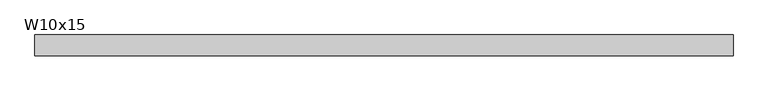
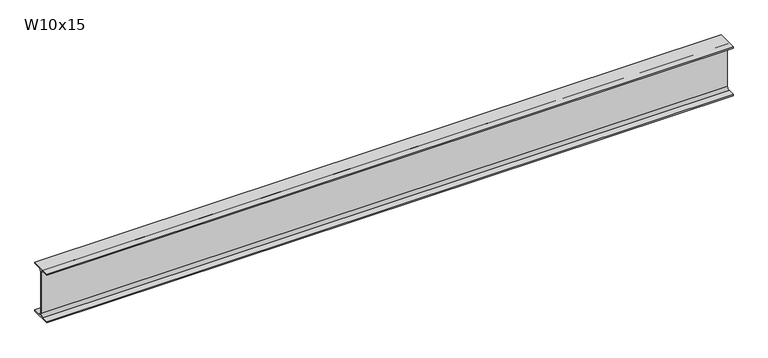
"""IFC4 building model written with IfcOpenShell, lengths in millimetres: beam geometry, RME W-Wide Flange : W10x15."""

from ifc_helpers import new_model, si_unit, point, frame, frame_2d, origin, place, context, project, spatial, polyline, circle_curve, trimmed, segment, composite_curve, outline, extrude, source, transform, mapped, element, save


def w10x15_0be6c648(model_context):
    return source(origin(), model_context, "Body", "SweptSolid", [
        extrude(outline(composite_curve([segment(polyline([(50.8, -120.142), (50.8, -127.0), (-50.8, -127.0), (-50.8, -120.142), (-16.7005, -120.142)]), True, "CONTINUOUS"), segment(trimmed(circle_curve(frame_2d((-16.7005, -106.3625)), 13.7795), [point((-16.7005, -120.142))], [point((-2.921, -106.3625))], True, "CARTESIAN"), True, "CONTINUOUS"), segment(polyline([(-2.921, -106.3625), (-2.921, 106.3625)]), True, "CONTINUOUS"), segment(trimmed(circle_curve(frame_2d((-16.7005, 106.3625)), 13.7795), [point((-2.921, 106.3625))], [point((-16.7005, 120.142))], True, "CARTESIAN"), True, "CONTINUOUS"), segment(polyline([(-16.7005, 120.142), (-50.8, 120.142), (-50.8, 127.0), (50.8, 127.0), (50.8, 120.142), (16.7005, 120.142)]), True, "CONTINUOUS"), segment(trimmed(circle_curve(frame_2d((16.7005, 106.3625)), 13.7795), [point((16.7005, 120.142))], [point((2.921, 106.3625))], True, "CARTESIAN"), True, "CONTINUOUS"), segment(polyline([(2.921, 106.3625), (2.921, -106.3625)]), True, "CONTINUOUS"), segment(trimmed(circle_curve(frame_2d((16.7005, -106.3625)), 13.7795), [point((2.921, -106.3625))], [point((16.7005, -120.142))], True, "CARTESIAN"), True, "CONTINUOUS"), segment(polyline([(16.7005, -120.142), (50.8, -120.142)]), True, "CONTINUOUS")], self_intersect=False)), frame((-1686.6702319, 0.0, 0.0), z_axis=(1.0, 0.0, 0.0), x_axis=(0.0, 1.0, 0.0)), (0.0, 0.0, 1.0), 3373.3404639),
    ])


if __name__ == "__main__":
    model = new_model("IFC4")
    model_context = context("Model", 3, world=origin())
    ifc_project = project(units=[si_unit("LENGTHUNIT", "METRE", prefix="MILLI")], contexts=[model_context])
    site = spatial("IfcSite", under=ifc_project)
    building = spatial("IfcBuilding", under=site)
    placement = place(None, origin())
    w10x15_shape = w10x15_0be6c648(model_context)
    element("IfcBeam", 1, ObjectType="RME W-Wide Flange : W10x15", at=placement, inside=building, context=model_context, shape_type="MappedRepresentation", body=[
        mapped(w10x15_shape, transform((0.0, 0.0, 0.0), x_axis=(1.0, 0.0, 0.0), y_axis=(0.0, 1.0, 0.0), z_axis=(0.0, 0.0, 1.0))),
    ])
    save(model, "model.ifc")

# Revit data of these elements
# Type "RME W-Wide Flange : W10x15"
#   WELD P [instance default] = ""
#   WELD LE [instance default] = ""
#   WELD D [instance default] = ""
#   TOP SECTION SIZE [instance default] = ""
#   TOP SECTION LENGTH [instance default] = ""
#   REMARKS [instance default] = ""
#   REINF TYPE [instance default] = ""
#   Nominal Size = "W24"
#   End Bearing Capacity [instance default] = ""
#   BOT SECTION SIZE [instance default] = ""
#   BOT SECTION LENGTH [instance default] = ""
#   Assembly Code = "B10"
#   W = 15
#   Start Extension Calculation [instance default] = 10' - 0"
#   Start Extension [instance default] = -0' - 0 1/2"
#   End Extension Calculation [instance default] = 10' - 0"
#   End Extension [instance default] = -0' - 0 1/2"
#   Length [instance default] = 5' - 0"
#   bf = 0' - 4"
#   d = 0' - 10"
#   k = 0' - 0 13/16"
#   k2 = 0' - 0.5425"
#   tf = 0' - 0.27"
#   tw = 0' - 0.23"
#   A = 0.030625 SF
#   Structural Material [instance default] = Metal - Steel - ASTM A992
# Element 1 (IfcBeam, "RME W-Wide Flange : W10x15")
#   Length = 11' - 0.80868"
#   Materials on its faces: "Metal - Steel - ASTM A992"
# Materials
#   "Metal - Steel - ASTM A992": class "Metal", colour RGB 255 128 0, transparency 0
